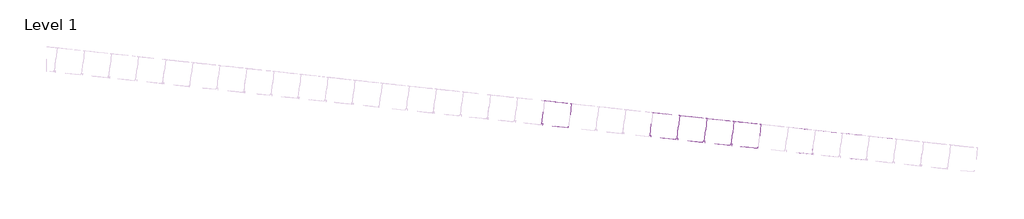
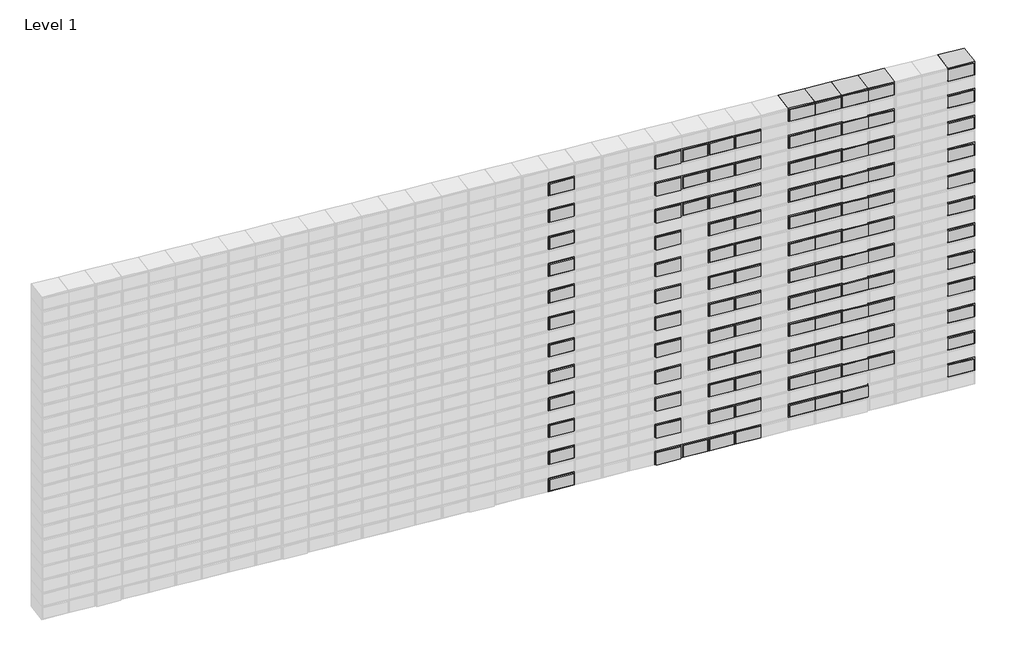
# One storey, part 17 of 18: 111 proxies.
"""IFC4 building model written with IfcOpenShell, lengths in millimetres."""

import ifcopenshell
import ifcopenshell.guid

model = None  # the IFC model being written
_history = None  # IfcOwnerHistory: only IFC2X3 demands one
_inside = {}  # id of a spatial element -> (the spatial element, [elements in it])
_under = {}  # id of a project, library or spatial element -> (it, [spatial elements below it])
_declared = {}  # id of a project -> (the project, [libraries it declares])
_typed = {}  # id of a type object -> (the type object, [elements of that type])
_made_of = {}  # id of a material, layer set ... -> (it, [elements and type objects made of it])


def new_model(schema):
    """Start an empty IFC model of exactly this schema.

    Asked for "IFC4X3", IfcOpenShell would pick the latest addendum, in which some entities
    have other attributes; the version numbers below select the first issue.
    IFC2X3 requires an IfcOwnerHistory on every rooted entity: one is made here for all.
    """
    global model, _history
    if schema == "IFC4X3":
        model = ifcopenshell.file(schema_version=(4, 3, 0, 0))
    else:
        model = ifcopenshell.file(schema=schema)
    _inside.clear()
    _under.clear()
    _declared.clear()
    _typed.clear()
    _made_of.clear()
    _history = None
    if model.schema == "IFC2X3":
        org = make("IfcOrganization", Name="unknown")
        user = make(
            "IfcPersonAndOrganization",
            ThePerson=make("IfcPerson", FamilyName="unknown"),
            TheOrganization=org,
        )
        app = make(
            "IfcApplication",
            ApplicationDeveloper=org,
            Version="unknown",
            ApplicationFullName="unknown",
            ApplicationIdentifier="unknown",
        )
        _history = make(
            "IfcOwnerHistory",
            OwningUser=user,
            OwningApplication=app,
            ChangeAction="ADDED",
            CreationDate=0,
        )
    return model


def make(cls, **values):
    """One entity of the class cls with the attributes given. An attribute that is None is left unset."""
    return model.create_entity(
        cls, **{name: value for name, value in values.items() if value is not None}
    )


def rooted(cls, **values):
    """An entity with a GlobalId (a new one), such as an element, a storey or a relation."""
    return make(cls, GlobalId=ifcopenshell.guid.new(), OwnerHistory=_history, **values)


def si_unit(unit_type, name, prefix=None):
    """IfcSIUnit, for example si_unit("LENGTHUNIT", "METRE", prefix="MILLI")."""
    return make("IfcSIUnit", UnitType=unit_type, Prefix=prefix, Name=name)


def assignment(units):
    """IfcUnitAssignment: the units of a project."""
    return None if units is None else make("IfcUnitAssignment", Units=units)


def point(xyz):
    """IfcCartesianPoint."""
    return None if xyz is None else make("IfcCartesianPoint", Coordinates=xyz)


def direction(xyz):
    """IfcDirection."""
    return None if xyz is None else make("IfcDirection", DirectionRatios=xyz)


def frame(location, z_axis=None, x_axis=None):
    """IfcAxis2Placement3D, a coordinate frame: its origin and axes. An axis left out is left unset."""
    return make(
        "IfcAxis2Placement3D",
        Location=point(location),
        Axis=direction(z_axis),
        RefDirection=direction(x_axis),
    )


def origin():
    """The frame at (0, 0, 0) with its axes left unset."""
    return frame((0.0, 0.0, 0.0))


def origin_with_axes():
    """The frame at (0, 0, 0) with the z axis (0, 0, 1) and the x axis (1, 0, 0) written out."""
    return frame((0.0, 0.0, 0.0), z_axis=(0.0, 0.0, 1.0), x_axis=(1.0, 0.0, 0.0))


def place(relative_to, where):
    """IfcLocalPlacement: puts the frame where relative to a parent placement (None: the world)."""
    return make(
        "IfcLocalPlacement", PlacementRelTo=relative_to, RelativePlacement=where
    )


def context(
    kind, dimensions, precision=None, world=None, true_north=None, identifier=None
):
    """IfcGeometricRepresentationContext, for example the 3D "Model" context."""
    return make(
        "IfcGeometricRepresentationContext",
        ContextIdentifier=identifier,
        ContextType=kind,
        CoordinateSpaceDimension=dimensions,
        Precision=precision,
        WorldCoordinateSystem=world,
        TrueNorth=true_north,
    )


def project(units=None, contexts=None):
    """IfcProject with its units and contexts."""
    return rooted(
        "IfcProject",
        Name="project",
        RepresentationContexts=contexts,
        UnitsInContext=assignment(units),
    )


def spatial(cls, under=None, at=None, **own):
    """A site, building, storey or space (cls), placed at a placement, below another one or the project."""
    s = rooted(cls, ObjectPlacement=at, **own)
    if under is not None:
        _under.setdefault(under.id(), (under, []))[1].append(s)
    return s


def polyline(points):
    """IfcPolyline through the points."""
    return make("IfcPolyline", Points=[point(p) for p in points])


def outline(outer, holes=None, kind="AREA"):
    """IfcArbitraryClosedProfileDef: a profile drawn as a closed curve; with holes, ...WithVoids."""
    if holes is None:
        return make("IfcArbitraryClosedProfileDef", ProfileType=kind, OuterCurve=outer)
    return make(
        "IfcArbitraryProfileDefWithVoids",
        ProfileType=kind,
        OuterCurve=outer,
        InnerCurves=holes,
    )


def extrude(swept, where, along, depth):
    """IfcExtrudedAreaSolid: the profile swept, set in the frame where, extruded along a direction by depth."""
    return make(
        "IfcExtrudedAreaSolid",
        SweptArea=swept,
        Position=where,
        ExtrudedDirection=direction(along),
        Depth=depth,
    )


def shape(context_of_items, identifier, shape_type, items):
    """IfcShapeRepresentation: the items that make up one representation, for example the "Body"."""
    return make(
        "IfcShapeRepresentation",
        ContextOfItems=context_of_items,
        RepresentationIdentifier=identifier,
        RepresentationType=shape_type,
        Items=items,
    )


def source(mapping_origin, context_of_items, identifier, shape_type, items):
    """IfcRepresentationMap: a shape defined once, which mapped items show again and again."""
    return make(
        "IfcRepresentationMap",
        MappingOrigin=mapping_origin,
        MappedRepresentation=shape(context_of_items, identifier, shape_type, items),
    )


def transform(
    local_origin,
    x_axis=None,
    y_axis=None,
    z_axis=None,
    scale=None,
    scale2=None,
    scale3=None,
    uniform=True,
):
    """IfcCartesianTransformationOperator3D, or its non-uniform kind. x_axis, y_axis, z_axis: its Axis1, 2, 3."""
    if uniform:
        return make(
            "IfcCartesianTransformationOperator3D",
            Axis1=direction(x_axis),
            Axis2=direction(y_axis),
            LocalOrigin=point(local_origin),
            Scale=scale,
            Axis3=direction(z_axis),
        )
    return make(
        "IfcCartesianTransformationOperator3DnonUniform",
        Axis1=direction(x_axis),
        Axis2=direction(y_axis),
        LocalOrigin=point(local_origin),
        Scale=scale,
        Axis3=direction(z_axis),
        Scale2=scale2,
        Scale3=scale3,
    )


def mapped(mapping_source, mapping_target):
    """IfcMappedItem: shows the shape of a source again, moved by a transform."""
    return make(
        "IfcMappedItem", MappingSource=mapping_source, MappingTarget=mapping_target
    )


def made_of(thing, what):
    """Note that an element or type object is made of a material, layer set ...; save() writes the relation."""
    if what is not None:
        _made_of.setdefault(what.id(), (what, []))[1].append(thing)
    return thing


def element(
    cls,
    number,
    at=None,
    inside=None,
    cuts=None,
    type_object=None,
    material=None,
    context=None,
    identifier="Body",
    shape_type=None,
    held_by="IfcProductDefinitionShape",
    body=None,
    shapes=None,
    **own,
):
    """One element of the class cls, such as IfcWall. Its Tag is "e" and its number.

    at: its placement. inside: the storey or other place that contains it. cuts: it is an
    opening in that element (IfcRelVoidsElement). A single representation is given by context,
    identifier, shape_type and body (its items); several are given by shapes. held_by: the class
    of the entity that holds the representations. save() writes the other relations.
    """
    e = rooted(cls, Tag="e%d" % number, ObjectPlacement=at, **own)
    if body is not None:
        shapes = [shape(context, identifier, shape_type, body)]
    if shapes is not None:
        e.Representation = make(held_by, Representations=shapes)
    if inside is not None:
        _inside.setdefault(inside.id(), (inside, []))[1].append(e)
    if cuts is not None:
        rooted(
            "IfcRelVoidsElement", RelatingBuildingElement=cuts, RelatedOpeningElement=e
        )
    if type_object is not None:
        _typed.setdefault(type_object.id(), (type_object, []))[1].append(e)
    return made_of(e, material)


def aggregate(whole, parts):
    """IfcRelAggregates: a whole, such as a stair, and the parts it consists of."""
    return rooted("IfcRelAggregates", RelatingObject=whole, RelatedObjects=parts)


def save(model, path):
    """Write the relations noted so far, then the file.

    IfcRelAggregates (storeys below a building ...), IfcRelContainedInSpatialStructure (elements
    in a storey), IfcRelDefinesByType, IfcRelAssociatesMaterial and IfcRelDeclares: one each for
    every whole, place, type object, material and project.
    """
    for whole, parts in _under.values():
        aggregate(whole, parts)
    for where, things in _inside.values():
        rooted(
            "IfcRelContainedInSpatialStructure",
            RelatedElements=things,
            RelatingStructure=where,
        )
    for kind, things in _typed.values():
        rooted("IfcRelDefinesByType", RelatedObjects=things, RelatingType=kind)
    for what, things in _made_of.values():
        rooted("IfcRelAssociatesMaterial", RelatedObjects=things, RelatingMaterial=what)
    for by, libraries in _declared.values():
        rooted("IfcRelDeclares", RelatingContext=by, RelatedDefinitions=libraries)
    model.write(path)


def geel_a5fc7152(model_context):
    return source(origin(), model_context, "Body", "SweptSolid", [
        extrude(outline(polyline([(131.1871262, 51.8695461), (24.8461542, 24.0369432), (23.5801491, 28.8740117), (125.0840527, 55.4406095), (111.9430518, 105.6488784), (10.4391482, 79.0822806), (9.1731432, 83.919349), (115.5141152, 111.7519519), (131.1871262, 51.8695461)])), origin_with_axes(), (0.0, 0.0, 1.0), 95.0),
        extrude(outline(polyline([(111.9430518, 105.6488784), (125.0840527, 55.4406095), (23.5801491, 28.8740117), (10.4391482, 79.0822806), (111.9430518, 105.6488784)])), origin_with_axes(), (0.0, 0.0, 1.0), 100.0),
    ])


def geel_ff5a4212(model_context):
    return source(origin(), model_context, "Body", "SweptSolid", [
        extrude(outline(polyline([(24.8461542, 24.0369432), (9.1731432, 83.919349), (115.5141152, 111.7519519), (116.7801202, 106.9148835), (15.2762167, 80.3482856), (28.4172176, 30.1400167), (129.9211211, 56.7066146), (131.1871262, 51.8695461), (24.8461542, 24.0369432)])), origin_with_axes(), (0.0, 0.0, 1.0), 95.0),
        extrude(outline(polyline([(116.7801202, 106.9148835), (129.9211211, 56.7066146), (28.4172176, 30.1400167), (15.2762167, 80.3482856), (116.7801202, 106.9148835)])), origin_with_axes(), (0.0, 0.0, 1.0), 100.0),
    ])


def rood_14a66368(model_context):
    return source(origin(), model_context, "Body", "SweptSolid", [
        extrude(outline(polyline([(24.8461542, 24.0369432), (9.1731432, 83.919349), (115.5141152, 111.7519519), (131.1871262, 51.8695461), (24.8461542, 24.0369432)]), holes=[polyline([(125.0840527, 55.4406095), (111.9430518, 105.6488784), (15.2762167, 80.3482856), (28.4172176, 30.1400167), (125.0840527, 55.4406095)])]), origin_with_axes(), (0.0, 0.0, 1.0), 95.0),
        extrude(outline(polyline([(111.9430518, 105.6488784), (125.0840527, 55.4406095), (28.4172176, 30.1400167), (15.2762167, 80.3482856), (111.9430518, 105.6488784)])), origin_with_axes(), (0.0, 0.0, 1.0), 100.0),
    ])


def rood_2ddd8018(model_context):
    return source(origin(), model_context, "Body", "SweptSolid", [
        extrude(outline(polyline([(24.8461542, 24.0369432), (9.1731432, 83.919349), (115.5141152, 111.7519519), (131.1871262, 51.8695461), (126.3500577, 50.6035411), (111.9430518, 105.6488784), (15.2762167, 80.3482856), (29.6832226, 25.3029482), (24.8461542, 24.0369432)])), origin_with_axes(), (0.0, 0.0, 1.0), 95.0),
        extrude(outline(polyline([(111.9430518, 105.6488784), (126.3500577, 50.6035411), (29.6832226, 25.3029482), (15.2762167, 80.3482856), (111.9430518, 105.6488784)])), origin_with_axes(), (0.0, 0.0, 1.0), 100.0),
    ])


model = new_model("IFC4")

# Units and contexts
model_context = context("Model", 3, world=origin())
ifc_project = project(units=[si_unit("LENGTHUNIT", "METRE", prefix="MILLI")], contexts=[model_context])

# Site, building, storey
site = spatial("IfcSite", under=ifc_project)
building = spatial("IfcBuilding", under=site)
storey = spatial("IfcBuildingStorey", under=building, Name="Level 1", Elevation=0.0)

# Proxies
placement = place(None, origin())
geel_shape = geel_a5fc7152(model_context)
element("IfcBuildingElementProxy", 1, Name="Geel", ObjectType="Geel", at=placement, inside=storey, context=model_context, shape_type="MappedRepresentation", body=[
    mapped(geel_shape, transform((12701.7798414, -4692.7839834, 2168.7358475), x_axis=(0.9617275503729374, -0.1047347566147725, -0.25320100633787673), y_axis=(0.25171277368869216, -0.02741220845642974, 0.9674136914420255), z_axis=(-0.10826263628609081, -0.9941223272738551, 0.0))),
])
element("IfcBuildingElementProxy", 2, Name="Geel", ObjectType="Geel", at=placement, inside=storey, context=model_context, shape_type="MappedRepresentation", body=[
    mapped(geel_shape, transform((12701.7798414, -4692.7839834, 2292.5348104), x_axis=(0.9617275503729374, -0.1047347566147725, -0.25320100633787673), y_axis=(0.25171277368869216, -0.02741220845642974, 0.9674136914420255), z_axis=(-0.10826263628609081, -0.9941223272738551, 0.0))),
])
element("IfcBuildingElementProxy", 3, Name="Geel", ObjectType="Geel", at=placement, inside=storey, context=model_context, shape_type="MappedRepresentation", body=[
    mapped(geel_shape, transform((12701.7798414, -4692.7839834, 2416.3337732), x_axis=(0.9617275503729384, -0.1047347566147726, -0.25320100633787307), y_axis=(0.25171277368868855, -0.02741220845642934, 0.9674136914420265), z_axis=(-0.10826263628609081, -0.994122327273855, 0.0))),
])
element("IfcBuildingElementProxy", 4, Name="Geel", ObjectType="Geel", at=placement, inside=storey, context=model_context, shape_type="MappedRepresentation", body=[
    mapped(geel_shape, transform((12701.7798414, -4692.7839834, 2540.132736), x_axis=(0.9617275503729374, -0.1047347566147725, -0.25320100633787673), y_axis=(0.25171277368869216, -0.02741220845642974, 0.9674136914420255), z_axis=(-0.10826263628609081, -0.9941223272738551, 0.0))),
])
element("IfcBuildingElementProxy", 5, Name="Geel", ObjectType="Geel", at=placement, inside=storey, context=model_context, shape_type="MappedRepresentation", body=[
    mapped(geel_shape, transform((12701.7798414, -4692.7839834, 2663.9316989), x_axis=(0.9617275503729374, -0.1047347566147725, -0.25320100633787673), y_axis=(0.25171277368869216, -0.02741220845642974, 0.9674136914420255), z_axis=(-0.10826263628609081, -0.9941223272738551, 0.0))),
])
element("IfcBuildingElementProxy", 6, Name="Geel", ObjectType="Geel", at=placement, inside=storey, context=model_context, shape_type="MappedRepresentation", body=[
    mapped(geel_shape, transform((12701.7798414, -4692.7839834, 2787.7306617), x_axis=(0.9617275503729374, -0.1047347566147725, -0.25320100633787673), y_axis=(0.25171277368869216, -0.02741220845642974, 0.9674136914420255), z_axis=(-0.10826263628609081, -0.9941223272738551, 0.0))),
])
element("IfcBuildingElementProxy", 7, Name="Geel", ObjectType="Geel", at=placement, inside=storey, context=model_context, shape_type="MappedRepresentation", body=[
    mapped(geel_shape, transform((12701.7798414, -4692.7839834, 2911.5296245), x_axis=(0.9617275503729374, -0.1047347566147725, -0.25320100633787673), y_axis=(0.25171277368869216, -0.02741220845642974, 0.9674136914420255), z_axis=(-0.10826263628609081, -0.9941223272738551, 0.0))),
])
element("IfcBuildingElementProxy", 8, Name="Geel", ObjectType="Geel", at=placement, inside=storey, context=model_context, shape_type="MappedRepresentation", body=[
    mapped(geel_shape, transform((12701.7798414, -4692.7839834, 3035.3285874), x_axis=(0.9617275503729374, -0.1047347566147725, -0.25320100633787673), y_axis=(0.25171277368869216, -0.02741220845642974, 0.9674136914420255), z_axis=(-0.10826263628609081, -0.9941223272738551, 0.0))),
])
element("IfcBuildingElementProxy", 9, Name="Geel", ObjectType="Geel", at=placement, inside=storey, context=model_context, shape_type="MappedRepresentation", body=[
    mapped(geel_shape, transform((12701.7798414, -4692.7839834, 3159.1275502), x_axis=(0.9617275503729374, -0.1047347566147725, -0.25320100633787673), y_axis=(0.25171277368869216, -0.02741220845642974, 0.9674136914420255), z_axis=(-0.10826263628609081, -0.9941223272738551, 0.0))),
])
element("IfcBuildingElementProxy", 10, Name="Geel", ObjectType="Geel", at=placement, inside=storey, context=model_context, shape_type="MappedRepresentation", body=[
    mapped(geel_shape, transform((12701.7798414, -4692.7839834, 3282.926513), x_axis=(0.9617275503729374, -0.1047347566147725, -0.25320100633787673), y_axis=(0.25171277368869216, -0.02741220845642974, 0.9674136914420255), z_axis=(-0.10826263628609081, -0.9941223272738551, 0.0))),
])
element("IfcBuildingElementProxy", 11, Name="Geel", ObjectType="Geel", at=placement, inside=storey, context=model_context, shape_type="MappedRepresentation", body=[
    mapped(geel_shape, transform((12701.7798414, -4692.7839834, 3406.7254759), x_axis=(0.9617275503729374, -0.1047347566147725, -0.25320100633787673), y_axis=(0.25171277368869216, -0.02741220845642974, 0.9674136914420255), z_axis=(-0.10826263628609081, -0.9941223272738551, 0.0))),
])
element("IfcBuildingElementProxy", 12, Name="Geel", ObjectType="Geel", at=placement, inside=storey, context=model_context, shape_type="MappedRepresentation", body=[
    mapped(geel_shape, transform((12701.7798414, -4692.7839834, 2044.9368847), x_axis=(0.9617275503729384, -0.1047347566147726, -0.25320100633787307), y_axis=(0.25171277368868855, -0.02741220845642934, 0.9674136914420265), z_axis=(-0.10826263628609081, -0.994122327273855, 0.0))),
])
element("IfcBuildingElementProxy", 13, Name="Geel", ObjectType="Geel", at=placement, inside=storey, context=model_context, shape_type="MappedRepresentation", body=[
    mapped(geel_shape, transform((12155.3955205, -4633.2812388, 2168.7358475), x_axis=(0.9617275503729422, -0.10473475661477022, -0.25320100633786), y_axis=(0.25171277368867573, -0.02741220845642721, 0.9674136914420299), z_axis=(-0.10826263628608798, -0.9941223272738554, 0.0))),
])
element("IfcBuildingElementProxy", 14, Name="Geel", ObjectType="Geel", at=placement, inside=storey, context=model_context, shape_type="MappedRepresentation", body=[
    mapped(geel_shape, transform((12155.3955205, -4633.2812388, 2292.5348104), x_axis=(0.9617275503729422, -0.10473475661477022, -0.25320100633786), y_axis=(0.25171277368867573, -0.02741220845642721, 0.9674136914420299), z_axis=(-0.10826263628608798, -0.9941223272738554, 0.0))),
])
element("IfcBuildingElementProxy", 15, Name="Geel", ObjectType="Geel", at=placement, inside=storey, context=model_context, shape_type="MappedRepresentation", body=[
    mapped(geel_shape, transform((12155.3955205, -4633.2812388, 2416.3337732), x_axis=(0.961727550372943, -0.10473475661477033, -0.25320100633785647), y_axis=(0.25171277368867206, -0.0274122084564268, 0.9674136914420309), z_axis=(-0.10826263628608797, -0.9941223272738553, 0.0))),
])
element("IfcBuildingElementProxy", 16, Name="Geel", ObjectType="Geel", at=placement, inside=storey, context=model_context, shape_type="MappedRepresentation", body=[
    mapped(geel_shape, transform((12155.3955205, -4633.2812388, 2540.132736), x_axis=(0.9617275503729422, -0.10473475661477022, -0.25320100633786), y_axis=(0.25171277368867573, -0.02741220845642721, 0.9674136914420299), z_axis=(-0.10826263628608798, -0.9941223272738554, 0.0))),
])
element("IfcBuildingElementProxy", 17, Name="Geel", ObjectType="Geel", at=placement, inside=storey, context=model_context, shape_type="MappedRepresentation", body=[
    mapped(geel_shape, transform((12155.3955205, -4633.2812388, 2663.9316989), x_axis=(0.9617275503729422, -0.10473475661477022, -0.25320100633786), y_axis=(0.25171277368867573, -0.02741220845642721, 0.9674136914420299), z_axis=(-0.10826263628608798, -0.9941223272738554, 0.0))),
])
element("IfcBuildingElementProxy", 18, Name="Geel", ObjectType="Geel", at=placement, inside=storey, context=model_context, shape_type="MappedRepresentation", body=[
    mapped(geel_shape, transform((12155.3955205, -4633.2812388, 2787.7306617), x_axis=(0.9617275503729422, -0.10473475661477022, -0.25320100633786), y_axis=(0.25171277368867573, -0.02741220845642721, 0.9674136914420299), z_axis=(-0.10826263628608798, -0.9941223272738554, 0.0))),
])
element("IfcBuildingElementProxy", 19, Name="Geel", ObjectType="Geel", at=placement, inside=storey, context=model_context, shape_type="MappedRepresentation", body=[
    mapped(geel_shape, transform((12155.3955205, -4633.2812388, 2911.5296245), x_axis=(0.9617275503729422, -0.10473475661477022, -0.25320100633786), y_axis=(0.25171277368867573, -0.02741220845642721, 0.9674136914420299), z_axis=(-0.10826263628608798, -0.9941223272738554, 0.0))),
])
element("IfcBuildingElementProxy", 20, Name="Geel", ObjectType="Geel", at=placement, inside=storey, context=model_context, shape_type="MappedRepresentation", body=[
    mapped(geel_shape, transform((12155.3955205, -4633.2812388, 3035.3285874), x_axis=(0.9617275503729422, -0.10473475661477022, -0.25320100633786), y_axis=(0.25171277368867573, -0.02741220845642721, 0.9674136914420299), z_axis=(-0.10826263628608798, -0.9941223272738554, 0.0))),
])
element("IfcBuildingElementProxy", 21, Name="Geel", ObjectType="Geel", at=placement, inside=storey, context=model_context, shape_type="MappedRepresentation", body=[
    mapped(geel_shape, transform((12155.3955205, -4633.2812388, 3159.1275502), x_axis=(0.9617275503729422, -0.10473475661477022, -0.25320100633786), y_axis=(0.25171277368867573, -0.02741220845642721, 0.9674136914420299), z_axis=(-0.10826263628608798, -0.9941223272738554, 0.0))),
])
element("IfcBuildingElementProxy", 22, Name="Geel", ObjectType="Geel", at=placement, inside=storey, context=model_context, shape_type="MappedRepresentation", body=[
    mapped(geel_shape, transform((12155.3955205, -4633.2812388, 3282.926513), x_axis=(0.9617275503729422, -0.10473475661477022, -0.25320100633786), y_axis=(0.25171277368867573, -0.02741220845642721, 0.9674136914420299), z_axis=(-0.10826263628608798, -0.9941223272738554, 0.0))),
])
element("IfcBuildingElementProxy", 23, Name="Geel", ObjectType="Geel", at=placement, inside=storey, context=model_context, shape_type="MappedRepresentation", body=[
    mapped(geel_shape, transform((12155.3955205, -4633.2812388, 3406.7254759), x_axis=(0.9617275503729422, -0.10473475661477022, -0.25320100633786), y_axis=(0.25171277368867573, -0.02741220845642721, 0.9674136914420299), z_axis=(-0.10826263628608798, -0.9941223272738554, 0.0))),
])
element("IfcBuildingElementProxy", 24, Name="Geel", ObjectType="Geel", at=placement, inside=storey, context=model_context, shape_type="MappedRepresentation", body=[
    mapped(geel_shape, transform((12155.3955205, -4633.2812388, 2044.9368847), x_axis=(0.961727550372943, -0.10473475661477033, -0.25320100633785647), y_axis=(0.25171277368867206, -0.0274122084564268, 0.9674136914420309), z_axis=(-0.10826263628608797, -0.9941223272738553, 0.0))),
])
element("IfcBuildingElementProxy", 25, Name="Geel", ObjectType="Geel", at=placement, inside=storey, context=model_context, shape_type="MappedRepresentation", body=[
    mapped(geel_shape, transform((12373.9492488, -4657.0823366, 2168.7358475), x_axis=(0.961727550372942, -0.1047347566147702, -0.25320100633786047), y_axis=(0.2517127736886762, -0.02741220845642727, 0.9674136914420297), z_axis=(-0.10826263628608798, -0.9941223272738554, 0.0))),
])
element("IfcBuildingElementProxy", 26, Name="Geel", ObjectType="Geel", at=placement, inside=storey, context=model_context, shape_type="MappedRepresentation", body=[
    mapped(geel_shape, transform((12373.9492488, -4657.0823366, 2292.5348104), x_axis=(0.961727550372942, -0.1047347566147702, -0.25320100633786047), y_axis=(0.2517127736886762, -0.02741220845642727, 0.9674136914420297), z_axis=(-0.10826263628608798, -0.9941223272738554, 0.0))),
])
element("IfcBuildingElementProxy", 27, Name="Geel", ObjectType="Geel", at=placement, inside=storey, context=model_context, shape_type="MappedRepresentation", body=[
    mapped(geel_shape, transform((12373.9492488, -4657.0823366, 2416.3337732), x_axis=(0.961727550372943, -0.10473475661477032, -0.25320100633785686), y_axis=(0.25171277368867245, -0.02741220845642687, 0.9674136914420308), z_axis=(-0.10826263628608798, -0.9941223272738553, 0.0))),
])
element("IfcBuildingElementProxy", 28, Name="Geel", ObjectType="Geel", at=placement, inside=storey, context=model_context, shape_type="MappedRepresentation", body=[
    mapped(geel_shape, transform((12373.9492488, -4657.0823366, 2540.132736), x_axis=(0.961727550372942, -0.1047347566147702, -0.25320100633786047), y_axis=(0.2517127736886762, -0.02741220845642727, 0.9674136914420297), z_axis=(-0.10826263628608798, -0.9941223272738554, 0.0))),
])
element("IfcBuildingElementProxy", 29, Name="Geel", ObjectType="Geel", at=placement, inside=storey, context=model_context, shape_type="MappedRepresentation", body=[
    mapped(geel_shape, transform((12373.9492488, -4657.0823366, 2663.9316989), x_axis=(0.961727550372942, -0.1047347566147702, -0.25320100633786047), y_axis=(0.2517127736886762, -0.02741220845642727, 0.9674136914420297), z_axis=(-0.10826263628608798, -0.9941223272738554, 0.0))),
])
element("IfcBuildingElementProxy", 30, Name="Geel", ObjectType="Geel", at=placement, inside=storey, context=model_context, shape_type="MappedRepresentation", body=[
    mapped(geel_shape, transform((12373.9492488, -4657.0823366, 2787.7306617), x_axis=(0.961727550372942, -0.1047347566147702, -0.25320100633786047), y_axis=(0.2517127736886762, -0.02741220845642727, 0.9674136914420297), z_axis=(-0.10826263628608798, -0.9941223272738554, 0.0))),
])
element("IfcBuildingElementProxy", 31, Name="Geel", ObjectType="Geel", at=placement, inside=storey, context=model_context, shape_type="MappedRepresentation", body=[
    mapped(geel_shape, transform((12373.9492488, -4657.0823366, 2911.5296245), x_axis=(0.961727550372942, -0.1047347566147702, -0.25320100633786047), y_axis=(0.2517127736886762, -0.02741220845642727, 0.9674136914420297), z_axis=(-0.10826263628608798, -0.9941223272738554, 0.0))),
])
element("IfcBuildingElementProxy", 32, Name="Geel", ObjectType="Geel", at=placement, inside=storey, context=model_context, shape_type="MappedRepresentation", body=[
    mapped(geel_shape, transform((12373.9492488, -4657.0823366, 3035.3285874), x_axis=(0.961727550372942, -0.1047347566147702, -0.25320100633786047), y_axis=(0.2517127736886762, -0.02741220845642727, 0.9674136914420297), z_axis=(-0.10826263628608798, -0.9941223272738554, 0.0))),
])
element("IfcBuildingElementProxy", 33, Name="Geel", ObjectType="Geel", at=placement, inside=storey, context=model_context, shape_type="MappedRepresentation", body=[
    mapped(geel_shape, transform((12373.9492488, -4657.0823366, 3159.1275502), x_axis=(0.961727550372942, -0.1047347566147702, -0.25320100633786047), y_axis=(0.2517127736886762, -0.02741220845642727, 0.9674136914420297), z_axis=(-0.10826263628608798, -0.9941223272738554, 0.0))),
])
element("IfcBuildingElementProxy", 34, Name="Geel", ObjectType="Geel", at=placement, inside=storey, context=model_context, shape_type="MappedRepresentation", body=[
    mapped(geel_shape, transform((12373.9492488, -4657.0823366, 3282.926513), x_axis=(0.961727550372942, -0.1047347566147702, -0.25320100633786047), y_axis=(0.2517127736886762, -0.02741220845642727, 0.9674136914420297), z_axis=(-0.10826263628608798, -0.9941223272738554, 0.0))),
])
element("IfcBuildingElementProxy", 35, Name="Geel", ObjectType="Geel", at=placement, inside=storey, context=model_context, shape_type="MappedRepresentation", body=[
    mapped(geel_shape, transform((12373.9492488, -4657.0823366, 3406.7254759), x_axis=(0.961727550372942, -0.1047347566147702, -0.25320100633786047), y_axis=(0.2517127736886762, -0.02741220845642727, 0.9674136914420297), z_axis=(-0.10826263628608798, -0.9941223272738554, 0.0))),
])
geel_2_shape = geel_ff5a4212(model_context)
element("IfcBuildingElementProxy", 36, Name="Geel", ObjectType="Geel", at=placement, inside=storey, context=model_context, shape_type="MappedRepresentation", body=[
    mapped(geel_2_shape, transform((12046.1186563, -4621.3806898, 2168.7358475), x_axis=(0.9617275503729374, -0.10473475661477244, -0.25320100633787673), y_axis=(0.25171277368869216, -0.02741220845642972, 0.9674136914420255), z_axis=(-0.10826263628609079, -0.9941223272738551, 0.0))),
])
element("IfcBuildingElementProxy", 37, Name="Geel", ObjectType="Geel", at=placement, inside=storey, context=model_context, shape_type="MappedRepresentation", body=[
    mapped(geel_2_shape, transform((12046.1186563, -4621.3806898, 2292.5348104), x_axis=(0.9617275503729374, -0.10473475661477244, -0.25320100633787673), y_axis=(0.25171277368869216, -0.02741220845642972, 0.9674136914420255), z_axis=(-0.10826263628609079, -0.9941223272738551, 0.0))),
])
element("IfcBuildingElementProxy", 38, Name="Geel", ObjectType="Geel", at=placement, inside=storey, context=model_context, shape_type="MappedRepresentation", body=[
    mapped(geel_2_shape, transform((12046.1186563, -4621.3806898, 2416.3337732), x_axis=(0.9617275503729384, -0.10473475661477256, -0.25320100633787307), y_axis=(0.25171277368868855, -0.02741220845642932, 0.9674136914420265), z_axis=(-0.10826263628609077, -0.994122327273855, 0.0))),
])
element("IfcBuildingElementProxy", 39, Name="Geel", ObjectType="Geel", at=placement, inside=storey, context=model_context, shape_type="MappedRepresentation", body=[
    mapped(geel_2_shape, transform((12046.1186563, -4621.3806898, 2540.132736), x_axis=(0.9617275503729374, -0.10473475661477244, -0.25320100633787673), y_axis=(0.25171277368869216, -0.02741220845642972, 0.9674136914420255), z_axis=(-0.10826263628609079, -0.9941223272738551, 0.0))),
])
element("IfcBuildingElementProxy", 40, Name="Geel", ObjectType="Geel", at=placement, inside=storey, context=model_context, shape_type="MappedRepresentation", body=[
    mapped(geel_2_shape, transform((12046.1186563, -4621.3806898, 2663.9316989), x_axis=(0.9617275503729374, -0.10473475661477244, -0.25320100633787673), y_axis=(0.25171277368869216, -0.02741220845642972, 0.9674136914420255), z_axis=(-0.10826263628609079, -0.9941223272738551, 0.0))),
])
element("IfcBuildingElementProxy", 41, Name="Geel", ObjectType="Geel", at=placement, inside=storey, context=model_context, shape_type="MappedRepresentation", body=[
    mapped(geel_2_shape, transform((12046.1186563, -4621.3806898, 2787.7306617), x_axis=(0.9617275503729374, -0.10473475661477244, -0.25320100633787673), y_axis=(0.25171277368869216, -0.02741220845642972, 0.9674136914420255), z_axis=(-0.10826263628609079, -0.9941223272738551, 0.0))),
])
element("IfcBuildingElementProxy", 42, Name="Geel", ObjectType="Geel", at=placement, inside=storey, context=model_context, shape_type="MappedRepresentation", body=[
    mapped(geel_2_shape, transform((12046.1186563, -4621.3806898, 2911.5296245), x_axis=(0.9617275503729374, -0.10473475661477244, -0.25320100633787673), y_axis=(0.25171277368869216, -0.02741220845642972, 0.9674136914420255), z_axis=(-0.10826263628609079, -0.9941223272738551, 0.0))),
])
element("IfcBuildingElementProxy", 43, Name="Geel", ObjectType="Geel", at=placement, inside=storey, context=model_context, shape_type="MappedRepresentation", body=[
    mapped(geel_2_shape, transform((12046.1186563, -4621.3806898, 3035.3285874), x_axis=(0.9617275503729374, -0.10473475661477244, -0.25320100633787673), y_axis=(0.25171277368869216, -0.02741220845642972, 0.9674136914420255), z_axis=(-0.10826263628609079, -0.9941223272738551, 0.0))),
])
element("IfcBuildingElementProxy", 44, Name="Geel", ObjectType="Geel", at=placement, inside=storey, context=model_context, shape_type="MappedRepresentation", body=[
    mapped(geel_2_shape, transform((12046.1186563, -4621.3806898, 3159.1275502), x_axis=(0.9617275503729374, -0.10473475661477244, -0.25320100633787673), y_axis=(0.25171277368869216, -0.02741220845642972, 0.9674136914420255), z_axis=(-0.10826263628609079, -0.9941223272738551, 0.0))),
])
element("IfcBuildingElementProxy", 45, Name="Geel", ObjectType="Geel", at=placement, inside=storey, context=model_context, shape_type="MappedRepresentation", body=[
    mapped(geel_2_shape, transform((12046.1186563, -4621.3806898, 3282.926513), x_axis=(0.9617275503729374, -0.10473475661477244, -0.25320100633787673), y_axis=(0.25171277368869216, -0.02741220845642972, 0.9674136914420255), z_axis=(-0.10826263628609079, -0.9941223272738551, 0.0))),
])
element("IfcBuildingElementProxy", 46, Name="Geel", ObjectType="Geel", at=placement, inside=storey, context=model_context, shape_type="MappedRepresentation", body=[
    mapped(geel_2_shape, transform((12046.1186563, -4621.3806898, 3406.7254759), x_axis=(0.9617275503729374, -0.10473475661477244, -0.25320100633787673), y_axis=(0.25171277368869216, -0.02741220845642972, 0.9674136914420255), z_axis=(-0.10826263628609079, -0.9941223272738551, 0.0))),
])
element("IfcBuildingElementProxy", 47, Name="Geel", ObjectType="Geel", at=placement, inside=storey, context=model_context, shape_type="MappedRepresentation", body=[
    mapped(geel_2_shape, transform((12046.1186563, -4621.3806898, 2044.9368847), x_axis=(0.9617275503729384, -0.10473475661477256, -0.25320100633787307), y_axis=(0.25171277368868855, -0.02741220845642932, 0.9674136914420265), z_axis=(-0.10826263628609077, -0.994122327273855, 0.0))),
])
element("IfcBuildingElementProxy", 48, Name="Geel", ObjectType="Geel", at=placement, inside=storey, context=model_context, shape_type="MappedRepresentation", body=[
    mapped(geel_2_shape, transform((12264.6723846, -4645.1817877, 2168.7358475), x_axis=(0.9617275503729374, -0.1047347566147725, -0.25320100633787673), y_axis=(0.25171277368869216, -0.02741220845642974, 0.9674136914420255), z_axis=(-0.10826263628609081, -0.9941223272738551, 0.0))),
])
element("IfcBuildingElementProxy", 49, Name="Geel", ObjectType="Geel", at=placement, inside=storey, context=model_context, shape_type="MappedRepresentation", body=[
    mapped(geel_2_shape, transform((12264.6723846, -4645.1817877, 2292.5348104), x_axis=(0.9617275503729374, -0.1047347566147725, -0.25320100633787673), y_axis=(0.25171277368869216, -0.02741220845642974, 0.9674136914420255), z_axis=(-0.10826263628609081, -0.9941223272738551, 0.0))),
])
element("IfcBuildingElementProxy", 50, Name="Geel", ObjectType="Geel", at=placement, inside=storey, context=model_context, shape_type="MappedRepresentation", body=[
    mapped(geel_2_shape, transform((12264.6723846, -4645.1817877, 2416.3337732), x_axis=(0.9617275503729384, -0.1047347566147726, -0.25320100633787307), y_axis=(0.25171277368868855, -0.02741220845642934, 0.9674136914420265), z_axis=(-0.10826263628609081, -0.994122327273855, 0.0))),
])
element("IfcBuildingElementProxy", 51, Name="Geel", ObjectType="Geel", at=placement, inside=storey, context=model_context, shape_type="MappedRepresentation", body=[
    mapped(geel_2_shape, transform((12264.6723846, -4645.1817877, 2540.132736), x_axis=(0.9617275503729374, -0.1047347566147725, -0.25320100633787673), y_axis=(0.25171277368869216, -0.02741220845642974, 0.9674136914420255), z_axis=(-0.10826263628609081, -0.9941223272738551, 0.0))),
])
element("IfcBuildingElementProxy", 52, Name="Geel", ObjectType="Geel", at=placement, inside=storey, context=model_context, shape_type="MappedRepresentation", body=[
    mapped(geel_2_shape, transform((12264.6723846, -4645.1817877, 2663.9316989), x_axis=(0.9617275503729374, -0.1047347566147725, -0.25320100633787673), y_axis=(0.25171277368869216, -0.02741220845642974, 0.9674136914420255), z_axis=(-0.10826263628609081, -0.9941223272738551, 0.0))),
])
element("IfcBuildingElementProxy", 53, Name="Geel", ObjectType="Geel", at=placement, inside=storey, context=model_context, shape_type="MappedRepresentation", body=[
    mapped(geel_2_shape, transform((12264.6723846, -4645.1817877, 2787.7306617), x_axis=(0.9617275503729374, -0.1047347566147725, -0.25320100633787673), y_axis=(0.25171277368869216, -0.02741220845642974, 0.9674136914420255), z_axis=(-0.10826263628609081, -0.9941223272738551, 0.0))),
])
element("IfcBuildingElementProxy", 54, Name="Geel", ObjectType="Geel", at=placement, inside=storey, context=model_context, shape_type="MappedRepresentation", body=[
    mapped(geel_2_shape, transform((12264.6723846, -4645.1817877, 2911.5296245), x_axis=(0.9617275503729374, -0.1047347566147725, -0.25320100633787673), y_axis=(0.25171277368869216, -0.02741220845642974, 0.9674136914420255), z_axis=(-0.10826263628609081, -0.9941223272738551, 0.0))),
])
element("IfcBuildingElementProxy", 55, Name="Geel", ObjectType="Geel", at=placement, inside=storey, context=model_context, shape_type="MappedRepresentation", body=[
    mapped(geel_2_shape, transform((12264.6723846, -4645.1817877, 3035.3285874), x_axis=(0.9617275503729374, -0.1047347566147725, -0.25320100633787673), y_axis=(0.25171277368869216, -0.02741220845642974, 0.9674136914420255), z_axis=(-0.10826263628609081, -0.9941223272738551, 0.0))),
])
element("IfcBuildingElementProxy", 56, Name="Geel", ObjectType="Geel", at=placement, inside=storey, context=model_context, shape_type="MappedRepresentation", body=[
    mapped(geel_2_shape, transform((12264.6723846, -4645.1817877, 3159.1275502), x_axis=(0.9617275503729374, -0.1047347566147725, -0.25320100633787673), y_axis=(0.25171277368869216, -0.02741220845642974, 0.9674136914420255), z_axis=(-0.10826263628609081, -0.9941223272738551, 0.0))),
])
element("IfcBuildingElementProxy", 57, Name="Geel", ObjectType="Geel", at=placement, inside=storey, context=model_context, shape_type="MappedRepresentation", body=[
    mapped(geel_2_shape, transform((12264.6723846, -4645.1817877, 3282.926513), x_axis=(0.9617275503729374, -0.1047347566147725, -0.25320100633787673), y_axis=(0.25171277368869216, -0.02741220845642974, 0.9674136914420255), z_axis=(-0.10826263628609081, -0.9941223272738551, 0.0))),
])
element("IfcBuildingElementProxy", 58, Name="Geel", ObjectType="Geel", at=placement, inside=storey, context=model_context, shape_type="MappedRepresentation", body=[
    mapped(geel_2_shape, transform((12264.6723846, -4645.1817877, 3406.7254759), x_axis=(0.9617275503729374, -0.1047347566147725, -0.25320100633787673), y_axis=(0.25171277368869216, -0.02741220845642974, 0.9674136914420255), z_axis=(-0.10826263628609081, -0.9941223272738551, 0.0))),
])
element("IfcBuildingElementProxy", 59, Name="Geel", ObjectType="Geel", at=placement, inside=storey, context=model_context, shape_type="MappedRepresentation", body=[
    mapped(geel_2_shape, transform((12264.6723846, -4645.1817877, 2044.9368847), x_axis=(0.9617275503729384, -0.1047347566147726, -0.25320100633787307), y_axis=(0.25171277368868855, -0.02741220845642934, 0.9674136914420265), z_axis=(-0.10826263628609081, -0.994122327273855, 0.0))),
])
rood_shape = rood_14a66368(model_context)
element("IfcBuildingElementProxy", 60, Name="Rood", ObjectType="Rood", at=placement, inside=storey, context=model_context, shape_type="MappedRepresentation", body=[
    mapped(rood_shape, transform((11609.0111995, -4573.7784941, 3097.2280688), x_axis=(0.9617275503729394, -0.10473475661477268, -0.2532010063378695), y_axis=(0.2517127736886849, -0.027412208456428923, 0.9674136914420275), z_axis=(-0.1082626362860908, -0.9941223272738551, 0.0))),
])
element("IfcBuildingElementProxy", 61, Name="Rood", ObjectType="Rood", at=placement, inside=storey, context=model_context, shape_type="MappedRepresentation", body=[
    mapped(rood_shape, transform((11609.0111995, -4573.7784941, 3221.0270316), x_axis=(0.9617275503729374, -0.1047347566147725, -0.25320100633787673), y_axis=(0.25171277368869216, -0.02741220845642974, 0.9674136914420255), z_axis=(-0.10826263628609081, -0.9941223272738551, 0.0))),
])
element("IfcBuildingElementProxy", 62, Name="Rood", ObjectType="Rood", at=placement, inside=storey, context=model_context, shape_type="MappedRepresentation", body=[
    mapped(rood_shape, transform((11609.0111995, -4573.7784941, 3344.8259944), x_axis=(0.9617275503729357, -0.10473475661477229, -0.2532010063378841), y_axis=(0.2517127736886993, -0.027412208456430498, 0.9674136914420237), z_axis=(-0.10826263628609081, -0.9941223272738551, 0.0))),
])
element("IfcBuildingElementProxy", 63, Name="Rood", ObjectType="Rood", at=placement, inside=storey, context=model_context, shape_type="MappedRepresentation", body=[
    mapped(rood_shape, transform((11609.0111995, -4573.7784941, 1983.0374033), x_axis=(0.9617275503729374, -0.1047347566147725, -0.25320100633787673), y_axis=(0.25171277368869216, -0.02741220845642974, 0.9674136914420255), z_axis=(-0.10826263628609081, -0.9941223272738551, 0.0))),
])
element("IfcBuildingElementProxy", 64, Name="Rood", ObjectType="Rood", at=placement, inside=storey, context=model_context, shape_type="MappedRepresentation", body=[
    mapped(rood_shape, transform((11718.2880637, -4585.679043, 2106.8363661), x_axis=(0.9617275503729374, -0.1047347566147725, -0.25320100633787673), y_axis=(0.25171277368869216, -0.02741220845642974, 0.9674136914420255), z_axis=(-0.10826263628609081, -0.9941223272738551, 0.0))),
])
element("IfcBuildingElementProxy", 65, Name="Rood", ObjectType="Rood", at=placement, inside=storey, context=model_context, shape_type="MappedRepresentation", body=[
    mapped(rood_shape, transform((11718.2880637, -4585.679043, 2230.6353289), x_axis=(0.9617275503729384, -0.1047347566147726, -0.25320100633787307), y_axis=(0.25171277368868855, -0.02741220845642934, 0.9674136914420265), z_axis=(-0.10826263628609081, -0.994122327273855, 0.0))),
])
element("IfcBuildingElementProxy", 66, Name="Rood", ObjectType="Rood", at=placement, inside=storey, context=model_context, shape_type="MappedRepresentation", body=[
    mapped(rood_shape, transform((11718.2880637, -4585.679043, 2354.4342918), x_axis=(0.9617275503729374, -0.1047347566147725, -0.25320100633787673), y_axis=(0.25171277368869216, -0.02741220845642974, 0.9674136914420255), z_axis=(-0.10826263628609081, -0.9941223272738551, 0.0))),
])
element("IfcBuildingElementProxy", 67, Name="Rood", ObjectType="Rood", at=placement, inside=storey, context=model_context, shape_type="MappedRepresentation", body=[
    mapped(rood_shape, transform((11718.2880637, -4585.679043, 2478.2332546), x_axis=(0.9617275503729374, -0.1047347566147725, -0.25320100633787673), y_axis=(0.25171277368869216, -0.02741220845642974, 0.9674136914420255), z_axis=(-0.10826263628609081, -0.9941223272738551, 0.0))),
])
element("IfcBuildingElementProxy", 68, Name="Rood", ObjectType="Rood", at=placement, inside=storey, context=model_context, shape_type="MappedRepresentation", body=[
    mapped(rood_shape, transform((11718.2880637, -4585.679043, 2602.0322174), x_axis=(0.9617275503729394, -0.10473475661477268, -0.2532010063378695), y_axis=(0.2517127736886849, -0.027412208456428923, 0.9674136914420275), z_axis=(-0.1082626362860908, -0.9941223272738551, 0.0))),
])
element("IfcBuildingElementProxy", 69, Name="Rood", ObjectType="Rood", at=placement, inside=storey, context=model_context, shape_type="MappedRepresentation", body=[
    mapped(rood_shape, transform((11718.2880637, -4585.679043, 2725.8311803), x_axis=(0.9617275503729374, -0.1047347566147725, -0.25320100633787673), y_axis=(0.25171277368869216, -0.02741220845642974, 0.9674136914420255), z_axis=(-0.10826263628609081, -0.9941223272738551, 0.0))),
])
element("IfcBuildingElementProxy", 70, Name="Rood", ObjectType="Rood", at=placement, inside=storey, context=model_context, shape_type="MappedRepresentation", body=[
    mapped(rood_shape, transform((11718.2880637, -4585.679043, 2849.6301431), x_axis=(0.9617275503729374, -0.1047347566147725, -0.25320100633787673), y_axis=(0.25171277368869216, -0.02741220845642974, 0.9674136914420255), z_axis=(-0.10826263628609081, -0.9941223272738551, 0.0))),
])
element("IfcBuildingElementProxy", 71, Name="Rood", ObjectType="Rood", at=placement, inside=storey, context=model_context, shape_type="MappedRepresentation", body=[
    mapped(rood_shape, transform((11718.2880637, -4585.679043, 2973.4291059), x_axis=(0.9617275503729374, -0.1047347566147725, -0.25320100633787673), y_axis=(0.25171277368869216, -0.02741220845642974, 0.9674136914420255), z_axis=(-0.10826263628609081, -0.9941223272738551, 0.0))),
])
element("IfcBuildingElementProxy", 72, Name="Rood", ObjectType="Rood", at=placement, inside=storey, context=model_context, shape_type="MappedRepresentation", body=[
    mapped(rood_shape, transform((11718.2880637, -4585.679043, 3097.2280688), x_axis=(0.9617275503729394, -0.10473475661477268, -0.2532010063378695), y_axis=(0.2517127736886849, -0.027412208456428923, 0.9674136914420275), z_axis=(-0.1082626362860908, -0.9941223272738551, 0.0))),
])
element("IfcBuildingElementProxy", 73, Name="Rood", ObjectType="Rood", at=placement, inside=storey, context=model_context, shape_type="MappedRepresentation", body=[
    mapped(rood_shape, transform((11718.2880637, -4585.679043, 3221.0270316), x_axis=(0.9617275503729374, -0.1047347566147725, -0.25320100633787673), y_axis=(0.25171277368869216, -0.02741220845642974, 0.9674136914420255), z_axis=(-0.10826263628609081, -0.9941223272738551, 0.0))),
])
element("IfcBuildingElementProxy", 74, Name="Rood", ObjectType="Rood", at=placement, inside=storey, context=model_context, shape_type="MappedRepresentation", body=[
    mapped(rood_shape, transform((11718.2880637, -4585.679043, 3344.8259944), x_axis=(0.9617275503729357, -0.10473475661477229, -0.2532010063378841), y_axis=(0.2517127736886993, -0.027412208456430498, 0.9674136914420237), z_axis=(-0.10826263628609081, -0.9941223272738551, 0.0))),
])
element("IfcBuildingElementProxy", 75, Name="Rood", ObjectType="Rood", at=placement, inside=storey, context=model_context, shape_type="MappedRepresentation", body=[
    mapped(rood_shape, transform((11718.2880637, -4585.679043, 1983.0374033), x_axis=(0.9617275503729374, -0.1047347566147725, -0.25320100633787673), y_axis=(0.25171277368869216, -0.02741220845642974, 0.9674136914420255), z_axis=(-0.10826263628609081, -0.9941223272738551, 0.0))),
])
element("IfcBuildingElementProxy", 76, Name="Rood", ObjectType="Rood", at=placement, inside=storey, context=model_context, shape_type="MappedRepresentation", body=[
    mapped(rood_shape, transform((11062.6268786, -4514.2757494, 2106.8363661), x_axis=(0.9617275503729374, -0.1047347566147725, -0.25320100633787673), y_axis=(0.25171277368869216, -0.02741220845642974, 0.9674136914420255), z_axis=(-0.10826263628609081, -0.9941223272738551, 0.0))),
])
element("IfcBuildingElementProxy", 77, Name="Rood", ObjectType="Rood", at=placement, inside=storey, context=model_context, shape_type="MappedRepresentation", body=[
    mapped(rood_shape, transform((11827.5649279, -4597.579592, 2106.8363661), x_axis=(0.9617275503729414, -0.10473475661477494, -0.25320100633786047), y_axis=(0.251712773688676, -0.027412208456428513, 0.9674136914420297), z_axis=(-0.10826263628609288, -0.9941223272738549, 0.0))),
])
element("IfcBuildingElementProxy", 78, Name="Rood", ObjectType="Rood", at=placement, inside=storey, context=model_context, shape_type="MappedRepresentation", body=[
    mapped(rood_shape, transform((11062.6268786, -4514.2757494, 2230.6353289), x_axis=(0.9617275503729384, -0.1047347566147726, -0.25320100633787307), y_axis=(0.25171277368868855, -0.02741220845642934, 0.9674136914420265), z_axis=(-0.10826263628609081, -0.994122327273855, 0.0))),
])
element("IfcBuildingElementProxy", 79, Name="Rood", ObjectType="Rood", at=placement, inside=storey, context=model_context, shape_type="MappedRepresentation", body=[
    mapped(rood_shape, transform((11827.5649279, -4597.579592, 2230.6353289), x_axis=(0.9617275503729424, -0.10473475661477503, -0.25320100633785697), y_axis=(0.25171277368867234, -0.027412208456428104, 0.9674136914420307), z_axis=(-0.10826263628609285, -0.9941223272738547, 0.0))),
])
element("IfcBuildingElementProxy", 80, Name="Rood", ObjectType="Rood", at=placement, inside=storey, context=model_context, shape_type="MappedRepresentation", body=[
    mapped(rood_shape, transform((11062.6268786, -4514.2757494, 2354.4342918), x_axis=(0.9617275503729374, -0.1047347566147725, -0.25320100633787673), y_axis=(0.25171277368869216, -0.02741220845642974, 0.9674136914420255), z_axis=(-0.10826263628609081, -0.9941223272738551, 0.0))),
])
element("IfcBuildingElementProxy", 81, Name="Rood", ObjectType="Rood", at=placement, inside=storey, context=model_context, shape_type="MappedRepresentation", body=[
    mapped(rood_shape, transform((11827.5649279, -4597.579592, 2354.4342918), x_axis=(0.9617275503729414, -0.10473475661477494, -0.25320100633786047), y_axis=(0.251712773688676, -0.027412208456428513, 0.9674136914420297), z_axis=(-0.10826263628609288, -0.9941223272738549, 0.0))),
])
element("IfcBuildingElementProxy", 82, Name="Rood", ObjectType="Rood", at=placement, inside=storey, context=model_context, shape_type="MappedRepresentation", body=[
    mapped(rood_shape, transform((11062.6268786, -4514.2757494, 2478.2332546), x_axis=(0.9617275503729374, -0.1047347566147725, -0.25320100633787673), y_axis=(0.25171277368869216, -0.02741220845642974, 0.9674136914420255), z_axis=(-0.10826263628609081, -0.9941223272738551, 0.0))),
])
element("IfcBuildingElementProxy", 83, Name="Rood", ObjectType="Rood", at=placement, inside=storey, context=model_context, shape_type="MappedRepresentation", body=[
    mapped(rood_shape, transform((11827.5649279, -4597.579592, 2478.2332546), x_axis=(0.9617275503729414, -0.10473475661477494, -0.25320100633786047), y_axis=(0.251712773688676, -0.027412208456428513, 0.9674136914420297), z_axis=(-0.10826263628609288, -0.9941223272738549, 0.0))),
])
element("IfcBuildingElementProxy", 84, Name="Rood", ObjectType="Rood", at=placement, inside=storey, context=model_context, shape_type="MappedRepresentation", body=[
    mapped(rood_shape, transform((11062.6268786, -4514.2757494, 2602.0322174), x_axis=(0.9617275503729394, -0.10473475661477268, -0.2532010063378695), y_axis=(0.2517127736886849, -0.027412208456428923, 0.9674136914420275), z_axis=(-0.1082626362860908, -0.9941223272738551, 0.0))),
])
element("IfcBuildingElementProxy", 85, Name="Rood", ObjectType="Rood", at=placement, inside=storey, context=model_context, shape_type="MappedRepresentation", body=[
    mapped(rood_shape, transform((11827.5649279, -4597.579592, 2602.0322174), x_axis=(0.9617275503729434, -0.10473475661477515, -0.2532010063378535), y_axis=(0.2517127736886688, -0.02741220845642771, 0.9674136914420317), z_axis=(-0.10826263628609288, -0.9941223272738549, 0.0))),
])
element("IfcBuildingElementProxy", 86, Name="Rood", ObjectType="Rood", at=placement, inside=storey, context=model_context, shape_type="MappedRepresentation", body=[
    mapped(rood_shape, transform((11062.6268786, -4514.2757494, 2725.8311803), x_axis=(0.9617275503729374, -0.1047347566147725, -0.25320100633787673), y_axis=(0.25171277368869216, -0.02741220845642974, 0.9674136914420255), z_axis=(-0.10826263628609081, -0.9941223272738551, 0.0))),
])
element("IfcBuildingElementProxy", 87, Name="Rood", ObjectType="Rood", at=placement, inside=storey, context=model_context, shape_type="MappedRepresentation", body=[
    mapped(rood_shape, transform((11827.5649279, -4597.579592, 2725.8311803), x_axis=(0.9617275503729414, -0.10473475661477494, -0.25320100633786047), y_axis=(0.251712773688676, -0.027412208456428513, 0.9674136914420297), z_axis=(-0.10826263628609288, -0.9941223272738549, 0.0))),
])
element("IfcBuildingElementProxy", 88, Name="Rood", ObjectType="Rood", at=placement, inside=storey, context=model_context, shape_type="MappedRepresentation", body=[
    mapped(rood_shape, transform((11062.6268786, -4514.2757494, 2849.6301431), x_axis=(0.9617275503729374, -0.1047347566147725, -0.25320100633787673), y_axis=(0.25171277368869216, -0.02741220845642974, 0.9674136914420255), z_axis=(-0.10826263628609081, -0.9941223272738551, 0.0))),
])
element("IfcBuildingElementProxy", 89, Name="Rood", ObjectType="Rood", at=placement, inside=storey, context=model_context, shape_type="MappedRepresentation", body=[
    mapped(rood_shape, transform((11827.5649279, -4597.579592, 2849.6301431), x_axis=(0.9617275503729414, -0.10473475661477494, -0.25320100633786047), y_axis=(0.251712773688676, -0.027412208456428513, 0.9674136914420297), z_axis=(-0.10826263628609288, -0.9941223272738549, 0.0))),
])
element("IfcBuildingElementProxy", 90, Name="Rood", ObjectType="Rood", at=placement, inside=storey, context=model_context, shape_type="MappedRepresentation", body=[
    mapped(rood_shape, transform((11062.6268786, -4514.2757494, 2973.4291059), x_axis=(0.9617275503729374, -0.1047347566147725, -0.25320100633787673), y_axis=(0.25171277368869216, -0.02741220845642974, 0.9674136914420255), z_axis=(-0.10826263628609081, -0.9941223272738551, 0.0))),
])
element("IfcBuildingElementProxy", 91, Name="Rood", ObjectType="Rood", at=placement, inside=storey, context=model_context, shape_type="MappedRepresentation", body=[
    mapped(rood_shape, transform((11827.5649279, -4597.579592, 2973.4291059), x_axis=(0.9617275503729414, -0.10473475661477494, -0.25320100633786047), y_axis=(0.251712773688676, -0.027412208456428513, 0.9674136914420297), z_axis=(-0.10826263628609288, -0.9941223272738549, 0.0))),
])
element("IfcBuildingElementProxy", 92, Name="Rood", ObjectType="Rood", at=placement, inside=storey, context=model_context, shape_type="MappedRepresentation", body=[
    mapped(rood_shape, transform((11062.6268786, -4514.2757494, 3097.2280688), x_axis=(0.9617275503729394, -0.10473475661477268, -0.2532010063378695), y_axis=(0.2517127736886849, -0.027412208456428923, 0.9674136914420275), z_axis=(-0.1082626362860908, -0.9941223272738551, 0.0))),
])
element("IfcBuildingElementProxy", 93, Name="Rood", ObjectType="Rood", at=placement, inside=storey, context=model_context, shape_type="MappedRepresentation", body=[
    mapped(rood_shape, transform((11827.5649279, -4597.579592, 3097.2280688), x_axis=(0.9617275503729434, -0.10473475661477515, -0.2532010063378535), y_axis=(0.2517127736886688, -0.02741220845642771, 0.9674136914420317), z_axis=(-0.10826263628609288, -0.9941223272738549, 0.0))),
])
element("IfcBuildingElementProxy", 94, Name="Rood", ObjectType="Rood", at=placement, inside=storey, context=model_context, shape_type="MappedRepresentation", body=[
    mapped(rood_shape, transform((11062.6268786, -4514.2757494, 3221.0270316), x_axis=(0.9617275503729374, -0.1047347566147725, -0.25320100633787673), y_axis=(0.25171277368869216, -0.02741220845642974, 0.9674136914420255), z_axis=(-0.10826263628609081, -0.9941223272738551, 0.0))),
])
element("IfcBuildingElementProxy", 95, Name="Rood", ObjectType="Rood", at=placement, inside=storey, context=model_context, shape_type="MappedRepresentation", body=[
    mapped(rood_shape, transform((11827.5649279, -4597.579592, 3221.0270316), x_axis=(0.9617275503729414, -0.10473475661477494, -0.25320100633786047), y_axis=(0.251712773688676, -0.027412208456428513, 0.9674136914420297), z_axis=(-0.10826263628609288, -0.9941223272738549, 0.0))),
])
element("IfcBuildingElementProxy", 96, Name="Rood", ObjectType="Rood", at=placement, inside=storey, context=model_context, shape_type="MappedRepresentation", body=[
    mapped(rood_shape, transform((11062.6268786, -4514.2757494, 3344.8259944), x_axis=(0.9617275503729357, -0.10473475661477229, -0.2532010063378841), y_axis=(0.2517127736886993, -0.027412208456430498, 0.9674136914420237), z_axis=(-0.10826263628609081, -0.9941223272738551, 0.0))),
])
element("IfcBuildingElementProxy", 97, Name="Rood", ObjectType="Rood", at=placement, inside=storey, context=model_context, shape_type="MappedRepresentation", body=[
    mapped(rood_shape, transform((11827.5649279, -4597.579592, 3344.8259944), x_axis=(0.9617275503729397, -0.10473475661477473, -0.2532010063378678), y_axis=(0.2517127736886832, -0.027412208456429284, 0.9674136914420279), z_axis=(-0.10826263628609287, -0.9941223272738549, 0.0))),
])
element("IfcBuildingElementProxy", 98, Name="Rood", ObjectType="Rood", at=placement, inside=storey, context=model_context, shape_type="MappedRepresentation", body=[
    mapped(rood_shape, transform((11062.6268786, -4514.2757494, 1983.0374033), x_axis=(0.9617275503729374, -0.1047347566147725, -0.25320100633787673), y_axis=(0.25171277368869216, -0.02741220845642974, 0.9674136914420255), z_axis=(-0.10826263628609081, -0.9941223272738551, 0.0))),
])
element("IfcBuildingElementProxy", 99, Name="Rood", ObjectType="Rood", at=placement, inside=storey, context=model_context, shape_type="MappedRepresentation", body=[
    mapped(rood_shape, transform((11827.5649279, -4597.579592, 1983.0374033), x_axis=(0.9617275503729414, -0.10473475661477494, -0.25320100633786047), y_axis=(0.251712773688676, -0.027412208456428513, 0.9674136914420297), z_axis=(-0.10826263628609288, -0.9941223272738549, 0.0))),
])
rood_2_shape = rood_2ddd8018(model_context)
element("IfcBuildingElementProxy", 100, Name="Rood", ObjectType="Rood", at=placement, inside=storey, context=model_context, shape_type="MappedRepresentation", body=[
    mapped(rood_2_shape, transform((11499.7343354, -4561.8779452, 1983.0374033), x_axis=(0.9617275503729381, -0.10473475661476775, -0.25320100633787634), y_axis=(0.2517127736886919, -0.02741220845642843, 0.9674136914420257), z_axis=(-0.1082626362860859, -0.9941223272738555, 0.0))),
])
element("IfcBuildingElementProxy", 101, Name="Rood", ObjectType="Rood", at=placement, inside=storey, context=model_context, shape_type="MappedRepresentation", body=[
    mapped(rood_2_shape, transform((11499.7343354, -4561.8779452, 2106.8363661), x_axis=(0.9617275503729381, -0.10473475661476775, -0.25320100633787634), y_axis=(0.2517127736886919, -0.02741220845642843, 0.9674136914420257), z_axis=(-0.1082626362860859, -0.9941223272738555, 0.0))),
])
element("IfcBuildingElementProxy", 102, Name="Rood", ObjectType="Rood", at=placement, inside=storey, context=model_context, shape_type="MappedRepresentation", body=[
    mapped(rood_2_shape, transform((11499.7343354, -4561.8779452, 2230.6353289), x_axis=(0.961727550372939, -0.10473475661476785, -0.2532010063378727), y_axis=(0.2517127736886882, -0.02741220845642804, 0.9674136914420266), z_axis=(-0.1082626362860859, -0.9941223272738555, 0.0))),
])
element("IfcBuildingElementProxy", 103, Name="Rood", ObjectType="Rood", at=placement, inside=storey, context=model_context, shape_type="MappedRepresentation", body=[
    mapped(rood_2_shape, transform((11499.7343354, -4561.8779452, 2354.4342918), x_axis=(0.9617275503729381, -0.10473475661476775, -0.25320100633787634), y_axis=(0.2517127736886919, -0.02741220845642843, 0.9674136914420257), z_axis=(-0.1082626362860859, -0.9941223272738555, 0.0))),
])
element("IfcBuildingElementProxy", 104, Name="Rood", ObjectType="Rood", at=placement, inside=storey, context=model_context, shape_type="MappedRepresentation", body=[
    mapped(rood_2_shape, transform((11499.7343354, -4561.8779452, 2478.2332546), x_axis=(0.9617275503729381, -0.10473475661476775, -0.25320100633787634), y_axis=(0.2517127736886919, -0.02741220845642843, 0.9674136914420257), z_axis=(-0.1082626362860859, -0.9941223272738555, 0.0))),
])
element("IfcBuildingElementProxy", 105, Name="Rood", ObjectType="Rood", at=placement, inside=storey, context=model_context, shape_type="MappedRepresentation", body=[
    mapped(rood_2_shape, transform((11499.7343354, -4561.8779452, 2602.0322174), x_axis=(0.96172755037294, -0.10473475661476794, -0.253201006337869), y_axis=(0.2517127736886847, -0.02741220845642766, 0.9674136914420275), z_axis=(-0.1082626362860859, -0.9941223272738556, 0.0))),
])
element("IfcBuildingElementProxy", 106, Name="Rood", ObjectType="Rood", at=placement, inside=storey, context=model_context, shape_type="MappedRepresentation", body=[
    mapped(rood_2_shape, transform((11499.7343354, -4561.8779452, 2725.8311803), x_axis=(0.9617275503729381, -0.10473475661476775, -0.25320100633787634), y_axis=(0.2517127736886919, -0.02741220845642843, 0.9674136914420257), z_axis=(-0.1082626362860859, -0.9941223272738555, 0.0))),
])
element("IfcBuildingElementProxy", 107, Name="Rood", ObjectType="Rood", at=placement, inside=storey, context=model_context, shape_type="MappedRepresentation", body=[
    mapped(rood_2_shape, transform((11499.7343354, -4561.8779452, 2849.6301431), x_axis=(0.9617275503729381, -0.10473475661476775, -0.25320100633787634), y_axis=(0.2517127736886919, -0.02741220845642843, 0.9674136914420257), z_axis=(-0.1082626362860859, -0.9941223272738555, 0.0))),
])
element("IfcBuildingElementProxy", 108, Name="Rood", ObjectType="Rood", at=placement, inside=storey, context=model_context, shape_type="MappedRepresentation", body=[
    mapped(rood_2_shape, transform((11499.7343354, -4561.8779452, 2973.4291059), x_axis=(0.9617275503729381, -0.10473475661476775, -0.25320100633787634), y_axis=(0.2517127736886919, -0.02741220845642843, 0.9674136914420257), z_axis=(-0.1082626362860859, -0.9941223272738555, 0.0))),
])
element("IfcBuildingElementProxy", 109, Name="Rood", ObjectType="Rood", at=placement, inside=storey, context=model_context, shape_type="MappedRepresentation", body=[
    mapped(rood_2_shape, transform((11499.7343354, -4561.8779452, 3097.2280688), x_axis=(0.96172755037294, -0.10473475661476794, -0.253201006337869), y_axis=(0.2517127736886847, -0.02741220845642766, 0.9674136914420275), z_axis=(-0.1082626362860859, -0.9941223272738556, 0.0))),
])
element("IfcBuildingElementProxy", 110, Name="Rood", ObjectType="Rood", at=placement, inside=storey, context=model_context, shape_type="MappedRepresentation", body=[
    mapped(rood_2_shape, transform((11499.7343354, -4561.8779452, 3221.0270316), x_axis=(0.9617275503729381, -0.10473475661476775, -0.25320100633787634), y_axis=(0.2517127736886919, -0.02741220845642843, 0.9674136914420257), z_axis=(-0.1082626362860859, -0.9941223272738555, 0.0))),
])
element("IfcBuildingElementProxy", 111, Name="Rood", ObjectType="Rood", at=placement, inside=storey, context=model_context, shape_type="MappedRepresentation", body=[
    mapped(rood_2_shape, transform((11499.7343354, -4561.8779452, 3344.8259944), x_axis=(0.9617275503729362, -0.10473475661476758, -0.2532010063378836), y_axis=(0.2517127736886991, -0.027412208456429242, 0.9674136914420237), z_axis=(-0.10826263628608593, -0.9941223272738555, 0.0))),
])

save(model, "model.ifc")

# Revit data of these elements
# Type "00_GMA_steen_versie_6 : Geel"
#   Voegdikte = 95 mm
#   VoegTovSteen = -5 mm
#   StootvoegLinksHalfOnder [instance default] = 5 mm
#   StootvoegLinksHalfBoven [instance default] = 5 mm
#   StootVoegRechtsHalfOnder [instance default] = 5 mm
#   StootVoegRechtsHalfBoven [instance default] = 5 mm
#   StootVoegBreedteRechts [instance default] = 10 mm
#   StootVoegBreedteLinks [instance default] = 10 mm
#   Steendikte = 100 mm
#   LintVoegOnderHalf [instance default] = 0 mm
#   LintVoegOnder [instance default] = 0 mm
#   LintVoegBovenHalf [instance default] = 5 mm
#   LintVoegBoven [instance default] = 10 mm
#   materiaal = 21_steen_geel
#   MateriaalVoeg = 20_voeg
#   Default Elevation = 0
# Type "00_GMA_steen_versie_6 : Rood"
#   Voegdikte = 95 mm
#   VoegTovSteen = -5 mm
#   StootvoegLinksHalfOnder [instance default] = 5 mm
#   StootvoegLinksHalfBoven [instance default] = 5 mm
#   StootVoegRechtsHalfOnder [instance default] = 5 mm
#   StootVoegRechtsHalfBoven [instance default] = 5 mm
#   StootVoegBreedteRechts [instance default] = 10 mm
#   StootVoegBreedteLinks [instance default] = 10 mm
#   Steendikte = 100 mm
#   LintVoegOnderHalf [instance default] = 0 mm
#   LintVoegOnder [instance default] = 0 mm
#   LintVoegBovenHalf [instance default] = 5 mm
#   LintVoegBoven [instance default] = 10 mm
#   materiaal = 21_steen_rood
#   MateriaalVoeg = 20_voeg
#   Default Elevation = 0
# Elements 1, 2, 3, 4, 5, 6, 7, 8, 9, 10, 11, 12, 13, 14, 15, 16, 17, 18, 19, 20, 21, 22, 23, 24, 25, 26, 27, 28, 29, 30, 31, 32, 33, 34, 35 (IfcBuildingElementProxy, "00_GMA_steen_versie_6 : Geel")
#   StootvoegLinksHalfOnder = 0 mm
#   StootvoegLinksHalfBoven = 0 mm
#   StootVoegRechtsHalfOnder = 5 mm
#   StootVoegRechtsHalfBoven = 5 mm
#   StootVoegBreedteRechts = 10 mm
#   StootVoegBreedteLinks = 0 mm
#   LintVoegOnderHalf = 5 mm
#   LintVoegOnder = 10 mm
#   LintVoegBovenHalf = 5 mm
#   LintVoegBoven = 10 mm
#   Phase Created = New Construction
#   Materials on its faces: "20_voeg", "21_steen_geel"
# Elements 36, 37, 38, 39, 40, 41, 42, 43, 44, 45, 46, 47, 48, 49, 50, 51, 52, 53, 54, 55, 56, 57, 58, 59 (IfcBuildingElementProxy, "00_GMA_steen_versie_6 : Geel")
#   StootvoegLinksHalfOnder = 5 mm
#   StootvoegLinksHalfBoven = 5 mm
#   StootVoegRechtsHalfOnder = 0 mm
#   StootVoegRechtsHalfBoven = 0 mm
#   StootVoegBreedteRechts = 0 mm
#   StootVoegBreedteLinks = 10 mm
#   LintVoegOnderHalf = 5 mm
#   LintVoegOnder = 10 mm
#   LintVoegBovenHalf = 5 mm
#   LintVoegBoven = 10 mm
